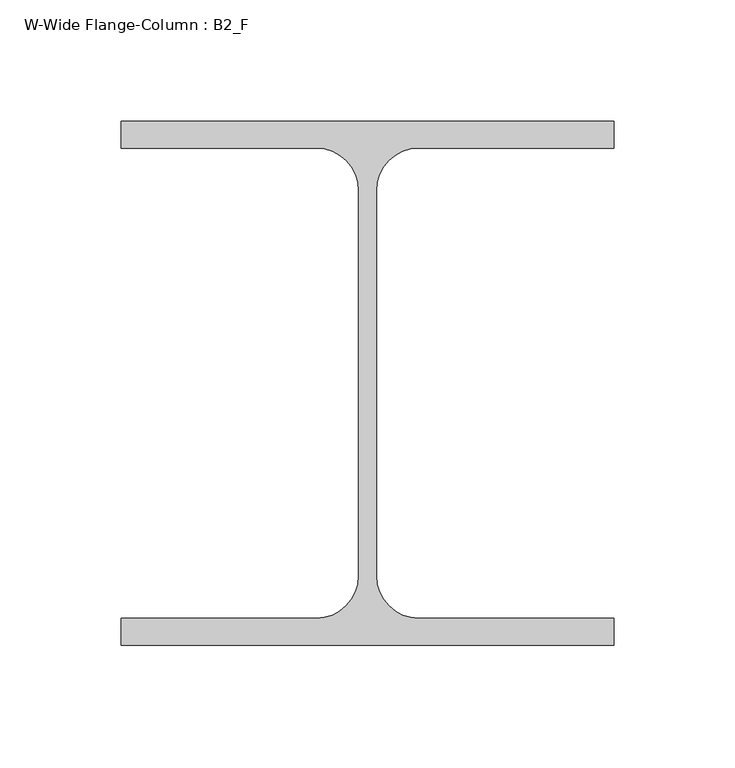
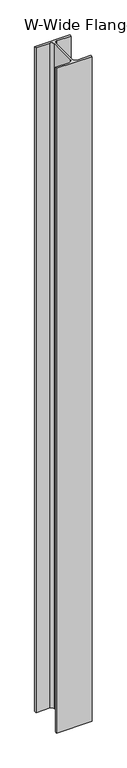
"""IFC4 building model written with IfcOpenShell, lengths in millimetres: column geometry, W-Wide Flange-Column : B2_F."""

from ifc_helpers import new_model, si_unit, point, frame, frame_2d, origin, place, context, project, spatial, polyline, circle_curve, trimmed, segment, composite_curve, outline, extrude, source, transform, mapped, element, save


def w_wide_flange_column_b2_f_fcbf751d(model_context):
    return source(origin(), model_context, "Body", "SweptSolid", [
        extrude(outline(composite_curve([segment(polyline([(101.6, 107.95), (101.6, 96.9367188), (21.2328125, 96.9367188)]), True, "CONTINUOUS"), segment(trimmed(circle_curve(frame_2d((21.2328125, 79.375)), 17.5617188), [point((21.2328125, 96.9367188))], [point((3.6710937, 79.375))], True, "CARTESIAN"), True, "CONTINUOUS"), segment(polyline([(3.6710937, 79.375), (3.6710937, -79.375)]), True, "CONTINUOUS"), segment(trimmed(circle_curve(frame_2d((21.2328125, -79.375)), 17.5617188), [point((3.6710937, -79.375))], [point((21.2328125, -96.9367187))], True, "CARTESIAN"), True, "CONTINUOUS"), segment(polyline([(21.2328125, -96.9367187), (101.6, -96.9367187), (101.6, -107.95), (-101.6, -107.95), (-101.6, -96.9367187), (-21.2328125, -96.9367187)]), True, "CONTINUOUS"), segment(trimmed(circle_curve(frame_2d((-21.2328125, -79.375)), 17.5617188), [point((-21.2328125, -96.9367187))], [point((-3.6710938, -79.375))], True, "CARTESIAN"), True, "CONTINUOUS"), segment(polyline([(-3.6710938, -79.375), (-3.6710938, 79.375)]), True, "CONTINUOUS"), segment(trimmed(circle_curve(frame_2d((-21.2328125, 79.375)), 17.5617188), [point((-3.6710938, 79.375))], [point((-21.2328125, 96.9367188))], True, "CARTESIAN"), True, "CONTINUOUS"), segment(polyline([(-21.2328125, 96.9367188), (-101.6, 96.9367188), (-101.6, 107.95), (101.6, 107.95)]), True, "CONTINUOUS")], self_intersect=False)), frame((0.0, 0.0, -304.8), z_axis=(0.0, 0.0, 1.0), x_axis=(1.0, 0.0, 0.0)), (0.0, 0.0, 1.0), 4025.9),
    ])


if __name__ == "__main__":
    model = new_model("IFC4")
    model_context = context("Model", 3, world=origin())
    ifc_project = project(units=[si_unit("LENGTHUNIT", "METRE", prefix="MILLI")], contexts=[model_context])
    site = spatial("IfcSite", under=ifc_project)
    building = spatial("IfcBuilding", under=site)
    placement = place(None, origin())
    w_wide_flange_column_b2_f_shape = w_wide_flange_column_b2_f_fcbf751d(model_context)
    element("IfcColumn", 1, ObjectType="W-Wide Flange-Column : B2_F", at=placement, inside=building, context=model_context, shape_type="MappedRepresentation", body=[
        mapped(w_wide_flange_column_b2_f_shape, transform((0.0, 0.0, 0.0), x_axis=(1.0, 0.0, 0.0), y_axis=(0.0, 1.0, 0.0), z_axis=(0.0, 0.0, 1.0))),
    ])
    save(model, "model.ifc")

# Revit data of these elements
# Type "W-Wide Flange-Column : B2_F"
#   Assembly Code = "B10"
#   W = 33
#   bf = 0' - 8"
#   d = 0' - 8 1/2"
#   k = 0' - 1 1/8"
#   kr = 0' - 0 177/256"
#   tf = 0' - 0 111/256"
#   tw = 0' - 0 37/128"
#   A = 0.07 SF
#   Structural Material [instance default] = Steel ASTM A992
# Element 1 (IfcColumn, "W-Wide Flange-Column : B2_F")
#   Structural Material = STRUCTURAL STEEL - SEE STRUCT. DWGS
#   Materials on its faces: "STRUCTURAL STEEL - SEE STRUCT. DWGS"
# Materials
#   "Steel ASTM A992": class "Metal", colour RGB 199 199 199, transparency 0, Description = "Structural steel 50ksi", Cost = 0
#   "STRUCTURAL STEEL - SEE STRUCT. DWGS": class "Metal", colour RGB 137 146 153, transparency 0, Description = "Steel, mill finish", Cost = 0
